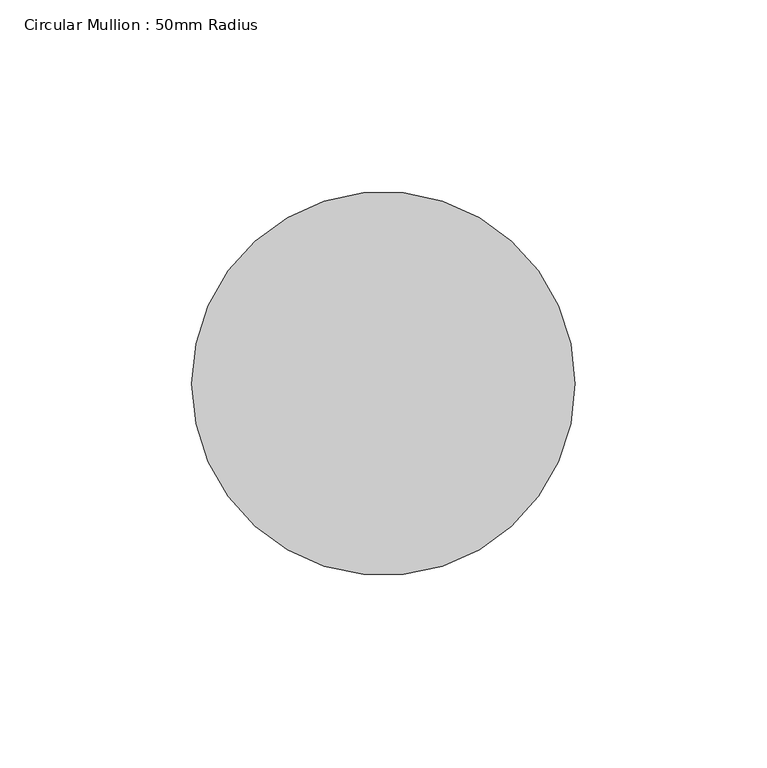
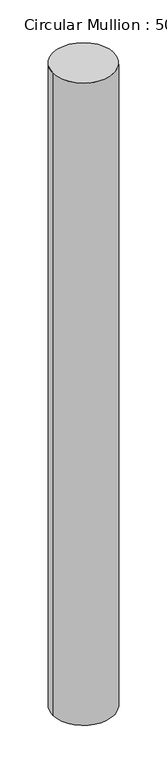
"""IFC4 building model written with IfcOpenShell, lengths in millimetres: member geometry, Circular Mullion : 50mm Radius."""

from ifc_helpers import new_model, si_unit, point, frame, origin, origin_2d, place, context, project, spatial, circle_curve, trimmed, segment, composite_curve, outline, extrude, source, transform, mapped, element, save


def circular_mullion_50mm_radius_3fdcc8d4(model_context):
    return source(origin(), model_context, "Body", "SweptSolid", [
        extrude(outline(composite_curve([segment(trimmed(circle_curve(origin_2d(), 50.0), [point((50.0, 0.0))], [point((-50.0, 0.0))], False, "CARTESIAN"), True, "CONTINUOUS"), segment(trimmed(circle_curve(origin_2d(), 50.0), [point((-50.0, 0.0))], [point((50.0, 0.0))], False, "CARTESIAN"), True, "CONTINUOUS")], self_intersect=False)), frame((0.0, 0.0, -1111.8499241), z_axis=(0.0, 0.0, 1.0), x_axis=(1.0, 0.0, 0.0)), (0.0, 0.0, 1.0), 1111.8499241),
    ])


if __name__ == "__main__":
    model = new_model("IFC4")
    model_context = context("Model", 3, world=origin())
    ifc_project = project(units=[si_unit("LENGTHUNIT", "METRE", prefix="MILLI")], contexts=[model_context])
    site = spatial("IfcSite", under=ifc_project)
    building = spatial("IfcBuilding", under=site)
    placement = place(None, origin())
    circular_mullion_50mm_radius_shape = circular_mullion_50mm_radius_3fdcc8d4(model_context)
    element("IfcMember", 1, ObjectType="Circular Mullion : 50mm Radius", at=placement, inside=building, context=model_context, shape_type="MappedRepresentation", body=[
        mapped(circular_mullion_50mm_radius_shape, transform((0.0, 0.0, 0.0), x_axis=(1.0, 0.0, 0.0), y_axis=(0.0, 1.0, 0.0), z_axis=(0.0, 0.0, 1.0))),
    ])
    save(model, "model.ifc")

# Revit data of these elements
# Type "Circular Mullion : 50mm Radius"
#   built-in parameter 1007350 = 0.164042 (stored number, unit not read)
# Element 1 (IfcMember, "Circular Mullion : 50mm Radius")
#   Materials on its faces: "Aluminium"
# Materials
#   "Aluminium": class "Metal", colour RGB 247 247 247, transparency 0, Description = "Aluminium 6061", Cost = 0
